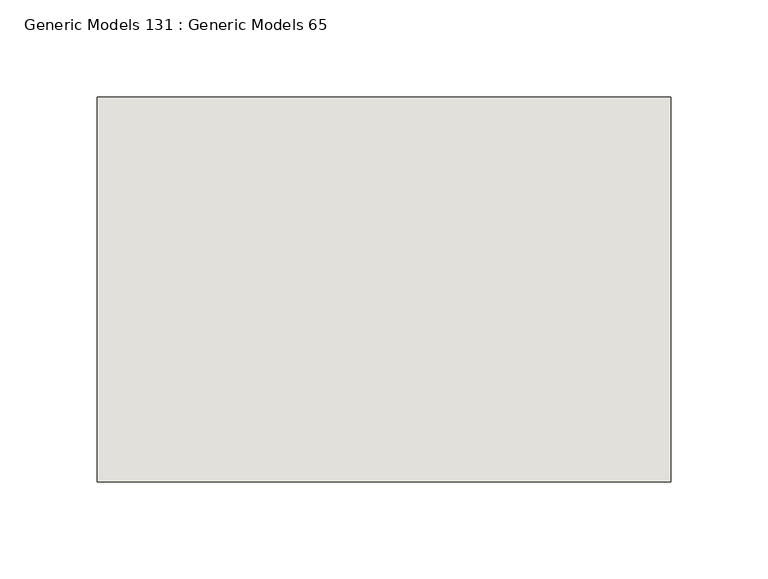
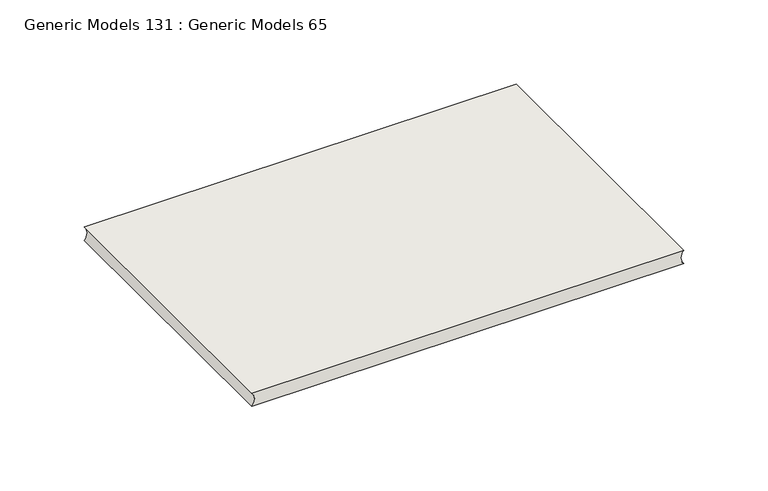
"""IFC4 building model written with IfcOpenShell, lengths in millimetres: wall geometry, Generic Models 131 : Generic Models 65."""

from ifc_helpers import new_model, si_unit, point, frame, frame_2d, origin, place, context, project, spatial, polyline, circle_curve, trimmed, segment, composite_curve, outline, extrude, source, transform, mapped, element, save


def generic_models_131_generic_models_65_4e516ed6(model_context):
    return source(origin(), model_context, "Body", "SweptSolid", [
        extrude(outline(composite_curve([segment(polyline([(1469.4712589, 375250.4413522), (1469.4712589, 374954.7151825)]), True, "CONTINUOUS"), segment(trimmed(circle_curve(frame_2d((1464.7087589, 374949.8321853)), 6.8209287), [point((1469.4712589, 374954.7151825))], [point((1459.9462589, 374954.7151825))], True, "CARTESIAN"), True, "CONTINUOUS"), segment(polyline([(1459.9462589, 374954.7151825), (1459.9462589, 375250.4413522)]), True, "CONTINUOUS"), segment(trimmed(circle_curve(frame_2d((1464.7087589, 375255.3243495)), 6.8209287), [point((1459.9462589, 375250.4413522))], [point((1469.4712589, 375250.4413522))], True, "CARTESIAN"), True, "CONTINUOUS")], self_intersect=False)), frame((0.0, 490.5375, 0.0), z_axis=(0.0, 1.0, 0.0), x_axis=(0.0, 0.0, 1.0)), (0.0, 0.0, 1.0), 198.4375),
    ])


if __name__ == "__main__":
    model = new_model("IFC4")
    model_context = context("Model", 3, world=origin())
    ifc_project = project(units=[si_unit("LENGTHUNIT", "METRE", prefix="MILLI")], contexts=[model_context])
    site = spatial("IfcSite", under=ifc_project)
    building = spatial("IfcBuilding", under=site)
    placement = place(None, origin())
    generic_models_131_generic_models_65_shape = generic_models_131_generic_models_65_4e516ed6(model_context)
    element("IfcWall", 1, ObjectType="Generic Models 131 : Generic Models 65", at=placement, inside=building, context=model_context, shape_type="MappedRepresentation", body=[
        mapped(generic_models_131_generic_models_65_shape, transform((0.0, 0.0, 0.0), x_axis=(1.0, 0.0, 0.0), y_axis=(0.0, 1.0, 0.0), z_axis=(0.0, 0.0, 1.0))),
    ])
    save(model, "model.ifc")

# Revit data of these elements
# Element 1 (IfcWall, "Generic Models 131 : Generic Models 65")
#   Materials on its faces: "MORTAR JOINT"
# Materials
#   "MORTAR JOINT": class "Generic", colour RGB 120 120 120, transparency 0, Cost = 0
